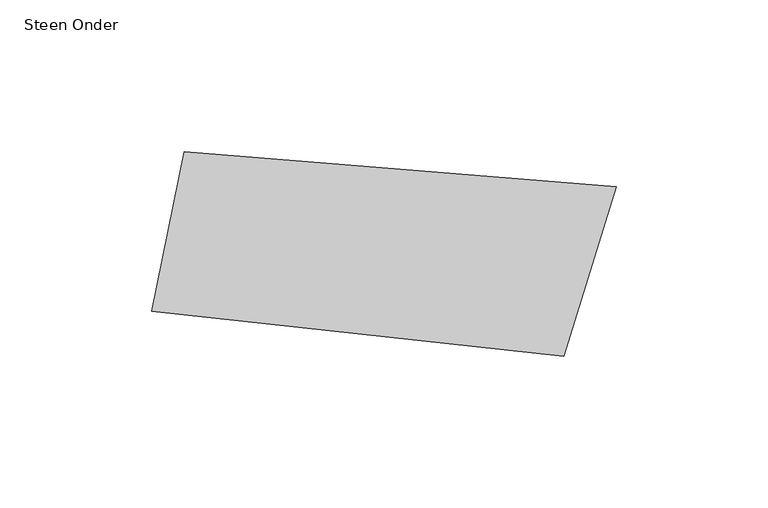
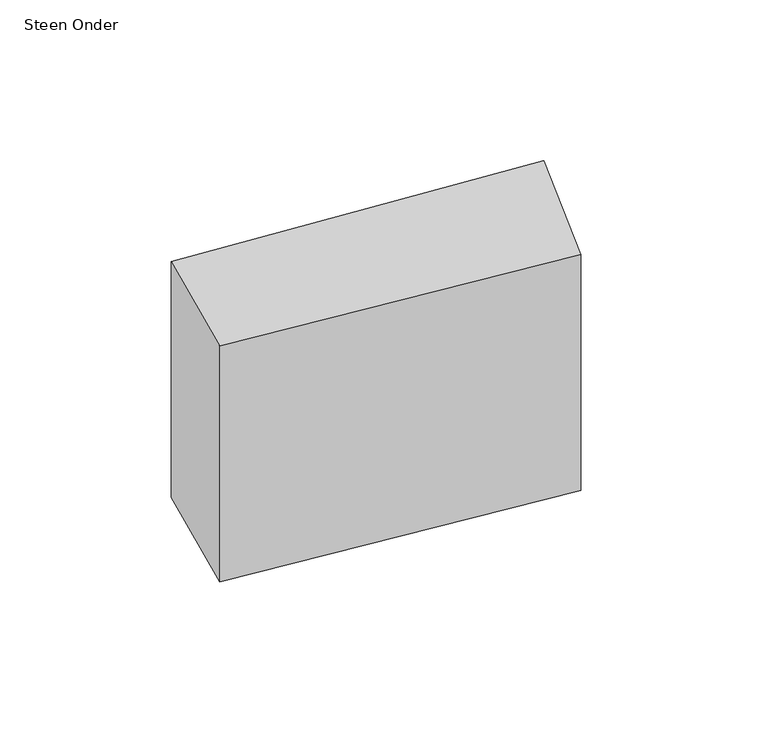
"""IFC4 building model written with IfcOpenShell, lengths in millimetres: proxy geometry, 00_GMA_steen_versie_4 : Steen Onder."""

from ifc_helpers import new_model, si_unit, frame, origin, place, context, project, spatial, polyline, outline, extrude, source, transform, mapped, element, save


def steen_onder_ecc8fdb5(model_context):
    return source(origin(), model_context, "Body", "SweptSolid", [
        extrude(outline(polyline([(173.2601072, 58.0986272), (155.9238451, 2.2847643), (19.8485661, 17.139288), (30.7074427, 69.7660302), (173.2601072, 58.0986272)])), frame((0.0, 0.0, -100.0), z_axis=(0.0, 0.0, 1.0), x_axis=(1.0, 0.0, 0.0)), (0.0, 0.0, 1.0), 100.0),
    ])


if __name__ == "__main__":
    model = new_model("IFC4")
    model_context = context("Model", 3, world=origin())
    ifc_project = project(units=[si_unit("LENGTHUNIT", "METRE", prefix="MILLI")], contexts=[model_context])
    site = spatial("IfcSite", under=ifc_project)
    building = spatial("IfcBuilding", under=site)
    placement = place(None, origin())
    steen_onder_shape = steen_onder_ecc8fdb5(model_context)
    element("IfcBuildingElementProxy", 1, Name="00_GMA_steen_versie_4 : Steen Onder", ObjectType="00_GMA_steen_versie_4 : Steen Onder", at=placement, inside=building, context=model_context, shape_type="MappedRepresentation", body=[
        mapped(steen_onder_shape, transform((0.0, 0.0, 0.0), x_axis=(1.0, 0.0, 0.0), y_axis=(0.0, 1.0, 0.0), z_axis=(0.0, 0.0, 1.0))),
    ])
    save(model, "model.ifc")

# Revit data of these elements
# Type "00_GMA_steen_versie_4 : Steen Onder"
#   StootVoegHalfBoven [instance default] = 5 mm
#   StootVoegHalf [instance default] = 5 mm
#   StootVoegBreedteOnder = 10 mm
#   StootVoegBreedteBoven = 10 mm
#   Steendikte = 100 mm
#   LintVoegOnderHalf = 0 mm
#   LintVoegOnder = 0 mm
#   LintVoegBovenHalf = 5 mm
#   LintVoegBoven = 10 mm
#   materiaal = none
#   MateriaalVoeg = none
#   Default Elevation = 0
